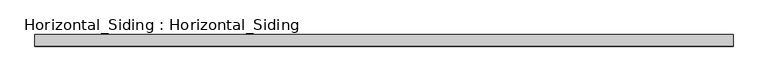
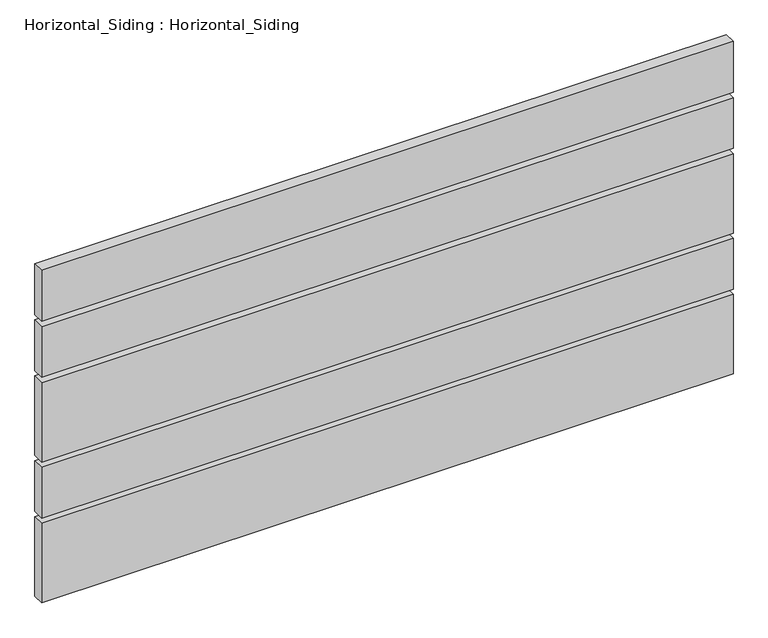
"""IFC4 building model written with IfcOpenShell, lengths in millimetres: plate geometry, Horizontal_Siding : Horizontal_Siding."""

from ifc_helpers import new_model, si_unit, frame, origin, place, context, project, spatial, polyline, outline, extrude, source, transform, mapped, element, save


def horizontal_siding_horizontal_siding_e22fd7a1(model_context):
    return source(origin(), model_context, "Body", "SweptSolid", [
        extrude(outline(polyline([(574.675, -19.05), (-574.675, -19.05), (-574.675, 0.0), (574.675, 0.0), (574.675, -19.05)])), frame((0.0, 0.0, 9.525), z_axis=(0.0, 0.0, 1.0), x_axis=(1.0, 0.0, 0.0)), (0.0, 0.0, 1.0), 139.7),
        extrude(outline(polyline([(574.675, -19.05), (-574.675, -19.05), (-574.675, 0.0), (574.675, 0.0), (574.675, -19.05)])), frame((0.0, 0.0, 158.75), z_axis=(0.0, 0.0, 1.0), x_axis=(1.0, 0.0, 0.0)), (0.0, 0.0, 1.0), 88.9),
        extrude(outline(polyline([(574.675, -19.05), (-574.675, -19.05), (-574.675, 0.0), (574.675, 0.0), (574.675, -19.05)])), frame((0.0, 0.0, 257.175), z_axis=(0.0, 0.0, 1.0), x_axis=(1.0, 0.0, 0.0)), (0.0, 0.0, 1.0), 139.7),
        extrude(outline(polyline([(574.675, -19.05), (-574.675, -19.05), (-574.675, 0.0), (574.675, 0.0), (574.675, -19.05)])), frame((0.0, 0.0, 406.4), z_axis=(0.0, 0.0, 1.0), x_axis=(1.0, 0.0, 0.0)), (0.0, 0.0, 1.0), 88.9),
        extrude(outline(polyline([(574.675, -19.05), (-574.675, -19.05), (-574.675, 0.0), (574.675, 0.0), (574.675, -19.05)])), frame((0.0, 0.0, 504.825), z_axis=(0.0, 0.0, 1.0), x_axis=(1.0, 0.0, 0.0)), (0.0, 0.0, 1.0), 88.9),
    ])


if __name__ == "__main__":
    model = new_model("IFC4")
    model_context = context("Model", 3, world=origin())
    ifc_project = project(units=[si_unit("LENGTHUNIT", "METRE", prefix="MILLI")], contexts=[model_context])
    site = spatial("IfcSite", under=ifc_project)
    building = spatial("IfcBuilding", under=site)
    placement = place(None, origin())
    horizontal_siding_horizontal_siding_shape = horizontal_siding_horizontal_siding_e22fd7a1(model_context)
    element("IfcPlate", 1, ObjectType="Horizontal_Siding : Horizontal_Siding", at=placement, inside=building, context=model_context, shape_type="MappedRepresentation", body=[
        mapped(horizontal_siding_horizontal_siding_shape, transform((0.0, 0.0, 0.0), x_axis=(1.0, 0.0, 0.0), y_axis=(0.0, 1.0, 0.0), z_axis=(0.0, 0.0, 1.0))),
    ])
    save(model, "model.ifc")

# Revit data of these elements
# Type "Horizontal_Siding : Horizontal_Siding"
#   Type Mark = "OUT"
#   Analytic Construction = "<None>"
#   extend = 0' - 2 3/4"
#   Width_2 = 0' - 3 1/2"
#   Width_1 = 0' - 5 1/2"
#   Gap = 0' - 0 3/8"
#   Plank Material = EXISTING HORZ. (1X4 & 1X6) WOOD SIDING (UNGROOVED PROFILE)
# Element 1 (IfcPlate, "Horizontal_Siding : Horizontal_Siding")
#   Materials on its faces: "EXISTING HORZ. (1X4 & 1X6) WOOD SIDING (UNGROOVED PROFILE)"
# Materials
#   "EXISTING HORZ. (1X4 & 1X6) WOOD SIDING (UNGROOVED PROFILE)": class "Wood", colour RGB 164 134 123, transparency 0, Description = "Pinus Echinata", Cost = 0
